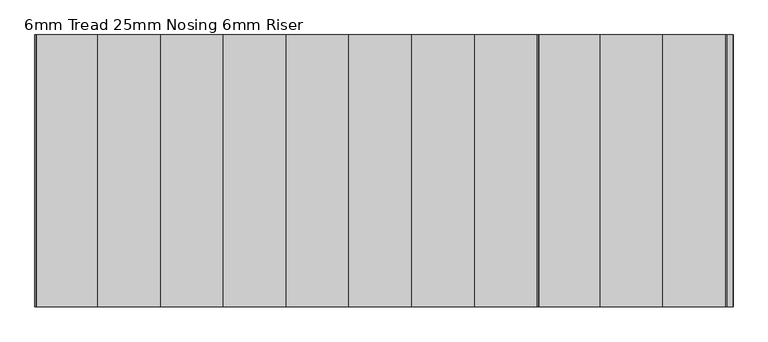
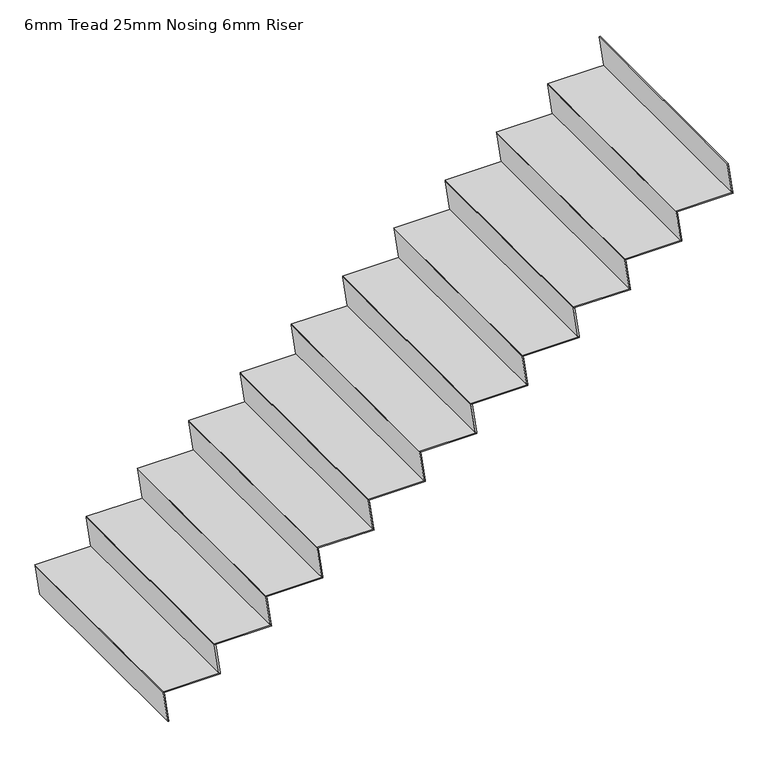
"""IFC4 building model written with IfcOpenShell, lengths in millimetres: stair flight geometry, 6mm Tread 25mm Nosing 6mm Riser."""

from ifc_helpers import new_model, si_unit, origin, place, context, project, spatial, faceted_brep, source, transform, mapped, element, save


def stair_flight_6mm_tread_25mm_nosing_6mm_riser_076b4cba(model_context):
    return source(origin(), model_context, "Body", "Brep", [
        faceted_brep([(-16043.9400908, 12030.4345331, 26529.4117647), (-16043.0900908, 12030.4345331, 26523.4117647), (-16043.0900908, 13220.4345331, 26523.4117647), (-16043.9400908, 13220.4345331, 26529.4117647), (-16350.0, 13220.4345331, 26529.4117647), (-16350.0, 12030.4345331, 26529.4117647), (-16349.15, 12030.4345331, 26523.4117647), (-16349.15, 13220.4345331, 26523.4117647)], [[[0, 1, 2, 3]], [[3, 4, 5, 0]], [[2, 1, 6, 7]], [[4, 3, 2, 7]], [[0, 5, 6, 1]], [[5, 4, 7, 6]]]),
        faceted_brep([(-16349.15, 12030.4345331, 26523.4117647), (-16325.0, 12030.4345331, 26352.9411765), (-16318.9400908, 12030.4345331, 26352.9411765), (-16343.0900908, 12030.4345331, 26523.4117647), (-16349.15, 13220.4345331, 26523.4117647), (-16343.0900908, 13220.4345331, 26523.4117647), (-16318.9400908, 13220.4345331, 26352.9411765), (-16325.0, 13220.4345331, 26352.9411765)], [[[0, 1, 2, 3]], [[4, 5, 6, 7]], [[1, 0, 4, 7]], [[2, 1, 7, 6]], [[3, 2, 6, 5]], [[0, 3, 5, 4]]]),
        faceted_brep([(-16074.15, 12030.4345331, 26699.8823529), (-16050.0, 12030.4345331, 26529.4117647), (-16043.9400908, 12030.4345331, 26529.4117647), (-16068.0900908, 12030.4345331, 26699.8823529), (-16074.15, 13220.4345331, 26699.8823529), (-16068.0900908, 13220.4345331, 26699.8823529), (-16043.9400908, 13220.4345331, 26529.4117647), (-16050.0, 13220.4345331, 26529.4117647)], [[[0, 1, 2, 3]], [[4, 5, 6, 7]], [[1, 0, 4, 7]], [[2, 1, 7, 6]], [[3, 2, 6, 5]], [[0, 3, 5, 4]]]),
        faceted_brep([(-15768.9400908, 13220.4345331, 26705.8823529), (-16075.0, 13220.4345331, 26705.8823529), (-16075.0, 12030.4345331, 26705.8823529), (-15768.9400908, 12030.4345331, 26705.8823529), (-15768.0900908, 13220.4345331, 26699.8823529), (-15768.0900908, 12030.4345331, 26699.8823529), (-16074.15, 12030.4345331, 26699.8823529), (-16074.15, 13220.4345331, 26699.8823529)], [[[0, 1, 2, 3]], [[4, 5, 6, 7]], [[1, 0, 4, 7]], [[3, 2, 6, 5]], [[3, 5, 4, 0]], [[2, 1, 7, 6]]]),
        faceted_brep([(-15799.15, 12030.4345331, 26876.3529412), (-15775.0, 12030.4345331, 26705.8823529), (-15768.9400908, 12030.4345331, 26705.8823529), (-15793.0900908, 12030.4345331, 26876.3529412), (-15799.15, 13220.4345331, 26876.3529412), (-15793.0900908, 13220.4345331, 26876.3529412), (-15768.9400908, 13220.4345331, 26705.8823529), (-15775.0, 13220.4345331, 26705.8823529)], [[[0, 1, 2, 3]], [[4, 5, 6, 7]], [[1, 0, 4, 7]], [[2, 1, 7, 6]], [[3, 2, 6, 5]], [[0, 3, 5, 4]]]),
        faceted_brep([(-15493.9400908, 13220.4345331, 26882.3529412), (-15800.0, 13220.4345331, 26882.3529412), (-15800.0, 12030.4345331, 26882.3529412), (-15493.9400908, 12030.4345331, 26882.3529412), (-15493.0900908, 13220.4345331, 26876.3529412), (-15493.0900908, 12030.4345331, 26876.3529412), (-15799.15, 12030.4345331, 26876.3529412), (-15799.15, 13220.4345331, 26876.3529412)], [[[0, 1, 2, 3]], [[4, 5, 6, 7]], [[1, 0, 4, 7]], [[3, 2, 6, 5]], [[3, 5, 4, 0]], [[2, 1, 7, 6]]]),
        faceted_brep([(-15524.15, 12030.4345331, 27052.8235294), (-15500.0, 12030.4345331, 26882.3529412), (-15493.9400908, 12030.4345331, 26882.3529412), (-15518.0900908, 12030.4345331, 27052.8235294), (-15524.15, 13220.4345331, 27052.8235294), (-15518.0900908, 13220.4345331, 27052.8235294), (-15493.9400908, 13220.4345331, 26882.3529412), (-15500.0, 13220.4345331, 26882.3529412)], [[[0, 1, 2, 3]], [[4, 5, 6, 7]], [[1, 0, 4, 7]], [[2, 1, 7, 6]], [[3, 2, 6, 5]], [[0, 3, 5, 4]]]),
        faceted_brep([(-15218.9400908, 13220.4345331, 27058.8235294), (-15525.0, 13220.4345331, 27058.8235294), (-15525.0, 12030.4345331, 27058.8235294), (-15218.9400908, 12030.4345331, 27058.8235294), (-15218.0900908, 13220.4345331, 27052.8235294), (-15218.0900908, 12030.4345331, 27052.8235294), (-15524.15, 12030.4345331, 27052.8235294), (-15524.15, 13220.4345331, 27052.8235294)], [[[0, 1, 2, 3]], [[4, 5, 6, 7]], [[1, 0, 4, 7]], [[3, 2, 6, 5]], [[3, 5, 4, 0]], [[2, 1, 7, 6]]]),
        faceted_brep([(-15249.15, 12030.4345331, 27229.2941176), (-15225.0, 12030.4345331, 27058.8235294), (-15218.9400908, 12030.4345331, 27058.8235294), (-15243.0900908, 12030.4345331, 27229.2941176), (-15249.15, 13220.4345331, 27229.2941176), (-15243.0900908, 13220.4345331, 27229.2941176), (-15218.9400908, 13220.4345331, 27058.8235294), (-15225.0, 13220.4345331, 27058.8235294)], [[[0, 1, 2, 3]], [[4, 5, 6, 7]], [[1, 0, 4, 7]], [[2, 1, 7, 6]], [[3, 2, 6, 5]], [[0, 3, 5, 4]]]),
        faceted_brep([(-14943.9400908, 13220.4345331, 27235.2941176), (-15250.0, 13220.4345331, 27235.2941176), (-15250.0, 12030.4345331, 27235.2941176), (-14943.9400908, 12030.4345331, 27235.2941176), (-14943.0900908, 13220.4345331, 27229.2941176), (-14943.0900908, 12030.4345331, 27229.2941176), (-15249.15, 12030.4345331, 27229.2941176), (-15249.15, 13220.4345331, 27229.2941176)], [[[0, 1, 2, 3]], [[4, 5, 6, 7]], [[1, 0, 4, 7]], [[3, 2, 6, 5]], [[3, 5, 4, 0]], [[2, 1, 7, 6]]]),
        faceted_brep([(-14974.15, 12030.4345331, 27405.7647059), (-14950.0, 12030.4345331, 27235.2941176), (-14943.9400908, 12030.4345331, 27235.2941176), (-14968.0900908, 12030.4345331, 27405.7647059), (-14974.15, 13220.4345331, 27405.7647059), (-14968.0900908, 13220.4345331, 27405.7647059), (-14943.9400908, 13220.4345331, 27235.2941176), (-14950.0, 13220.4345331, 27235.2941176)], [[[0, 1, 2, 3]], [[4, 5, 6, 7]], [[1, 0, 4, 7]], [[2, 1, 7, 6]], [[3, 2, 6, 5]], [[0, 3, 5, 4]]]),
        faceted_brep([(-14668.9400908, 13220.4345331, 27411.7647059), (-14975.0, 13220.4345331, 27411.7647059), (-14975.0, 12030.4345331, 27411.7647059), (-14668.9400908, 12030.4345331, 27411.7647059), (-14668.0900908, 13220.4345331, 27405.7647059), (-14668.0900908, 12030.4345331, 27405.7647059), (-14974.15, 12030.4345331, 27405.7647059), (-14974.15, 13220.4345331, 27405.7647059)], [[[0, 1, 2, 3]], [[4, 5, 6, 7]], [[1, 0, 4, 7]], [[3, 2, 6, 5]], [[3, 5, 4, 0]], [[2, 1, 7, 6]]]),
        faceted_brep([(-14699.15, 12030.4345331, 27582.2352941), (-14675.0, 12030.4345331, 27411.7647059), (-14668.9400908, 12030.4345331, 27411.7647059), (-14693.0900908, 12030.4345331, 27582.2352941), (-14699.15, 13220.4345331, 27582.2352941), (-14693.0900908, 13220.4345331, 27582.2352941), (-14668.9400908, 13220.4345331, 27411.7647059), (-14675.0, 13220.4345331, 27411.7647059)], [[[0, 1, 2, 3]], [[4, 5, 6, 7]], [[1, 0, 4, 7]], [[2, 1, 7, 6]], [[3, 2, 6, 5]], [[0, 3, 5, 4]]]),
        faceted_brep([(-14393.9400908, 13220.4345331, 27588.2352941), (-14700.0, 13220.4345331, 27588.2352941), (-14700.0, 12030.4345331, 27588.2352941), (-14393.9400908, 12030.4345331, 27588.2352941), (-14393.0900908, 13220.4345331, 27582.2352941), (-14393.0900908, 12030.4345331, 27582.2352941), (-14699.15, 12030.4345331, 27582.2352941), (-14699.15, 13220.4345331, 27582.2352941)], [[[0, 1, 2, 3]], [[4, 5, 6, 7]], [[1, 0, 4, 7]], [[3, 2, 6, 5]], [[3, 5, 4, 0]], [[2, 1, 7, 6]]]),
        faceted_brep([(-14424.15, 12030.4345331, 27758.7058824), (-14400.0, 12030.4345331, 27588.2352941), (-14393.9400908, 12030.4345331, 27588.2352941), (-14418.0900908, 12030.4345331, 27758.7058824), (-14424.15, 13220.4345331, 27758.7058824), (-14418.0900908, 13220.4345331, 27758.7058824), (-14393.9400908, 13220.4345331, 27588.2352941), (-14400.0, 13220.4345331, 27588.2352941)], [[[0, 1, 2, 3]], [[4, 5, 6, 7]], [[1, 0, 4, 7]], [[2, 1, 7, 6]], [[3, 2, 6, 5]], [[0, 3, 5, 4]]]),
        faceted_brep([(-14118.9400908, 13220.4345331, 27764.7058824), (-14425.0, 13220.4345331, 27764.7058824), (-14425.0, 12030.4345331, 27764.7058824), (-14118.9400908, 12030.4345331, 27764.7058824), (-14118.0900908, 13220.4345331, 27758.7058824), (-14118.0900908, 12030.4345331, 27758.7058824), (-14424.15, 12030.4345331, 27758.7058824), (-14424.15, 13220.4345331, 27758.7058824)], [[[0, 1, 2, 3]], [[4, 5, 6, 7]], [[1, 0, 4, 7]], [[3, 2, 6, 5]], [[3, 5, 4, 0]], [[2, 1, 7, 6]]]),
        faceted_brep([(-14149.15, 12030.4345331, 27935.1764706), (-14125.0, 12030.4345331, 27764.7058824), (-14118.9400908, 12030.4345331, 27764.7058824), (-14143.0900908, 12030.4345331, 27935.1764706), (-14149.15, 13220.4345331, 27935.1764706), (-14143.0900908, 13220.4345331, 27935.1764706), (-14118.9400908, 13220.4345331, 27764.7058824), (-14125.0, 13220.4345331, 27764.7058824)], [[[0, 1, 2, 3]], [[4, 5, 6, 7]], [[1, 0, 4, 7]], [[2, 1, 7, 6]], [[3, 2, 6, 5]], [[0, 3, 5, 4]]]),
        faceted_brep([(-13843.9400908, 13220.4345331, 27941.1764706), (-14150.0, 13220.4345331, 27941.1764706), (-14150.0, 12030.4345331, 27941.1764706), (-13843.9400908, 12030.4345331, 27941.1764706), (-13843.0900908, 13220.4345331, 27935.1764706), (-13843.0900908, 12030.4345331, 27935.1764706), (-14149.15, 12030.4345331, 27935.1764706), (-14149.15, 13220.4345331, 27935.1764706)], [[[0, 1, 2, 3]], [[4, 5, 6, 7]], [[1, 0, 4, 7]], [[3, 2, 6, 5]], [[3, 5, 4, 0]], [[2, 1, 7, 6]]]),
        faceted_brep([(-13874.15, 12030.4345331, 28111.6470588), (-13850.0, 12030.4345331, 27941.1764706), (-13843.9400908, 12030.4345331, 27941.1764706), (-13868.0900908, 12030.4345331, 28111.6470588), (-13874.15, 13220.4345331, 28111.6470588), (-13868.0900908, 13220.4345331, 28111.6470588), (-13843.9400908, 13220.4345331, 27941.1764706), (-13850.0, 13220.4345331, 27941.1764706)], [[[0, 1, 2, 3]], [[4, 5, 6, 7]], [[1, 0, 4, 7]], [[2, 1, 7, 6]], [[3, 2, 6, 5]], [[0, 3, 5, 4]]]),
        faceted_brep([(-13568.9400908, 13220.4345331, 28117.6470588), (-13875.0, 13220.4345331, 28117.6470588), (-13875.0, 12030.4345331, 28117.6470588), (-13568.9400908, 12030.4345331, 28117.6470588), (-13568.0900908, 13220.4345331, 28111.6470588), (-13568.0900908, 12030.4345331, 28111.6470588), (-13874.15, 12030.4345331, 28111.6470588), (-13874.15, 13220.4345331, 28111.6470588)], [[[0, 1, 2, 3]], [[4, 5, 6, 7]], [[1, 0, 4, 7]], [[3, 2, 6, 5]], [[3, 5, 4, 0]], [[2, 1, 7, 6]]]),
        faceted_brep([(-13324.15, 12030.4345331, 28464.5882353), (-13300.0, 12030.4345331, 28294.1176471), (-13293.9400908, 12030.4345331, 28294.1176471), (-13318.0900908, 12030.4345331, 28464.5882353), (-13324.15, 13220.4345331, 28464.5882353), (-13318.0900908, 13220.4345331, 28464.5882353), (-13293.9400908, 13220.4345331, 28294.1176471), (-13300.0, 13220.4345331, 28294.1176471)], [[[0, 1, 2, 3]], [[4, 5, 6, 7]], [[1, 0, 4, 7]], [[2, 1, 7, 6]], [[3, 2, 6, 5]], [[0, 3, 5, 4]]]),
        faceted_brep([(-13599.15, 12030.4345331, 28288.1176471), (-13575.0, 12030.4345331, 28117.6470588), (-13568.9400908, 12030.4345331, 28117.6470588), (-13593.0900908, 12030.4345331, 28288.1176471), (-13599.15, 13220.4345331, 28288.1176471), (-13593.0900908, 13220.4345331, 28288.1176471), (-13568.9400908, 13220.4345331, 28117.6470588), (-13575.0, 13220.4345331, 28117.6470588)], [[[0, 1, 2, 3]], [[4, 5, 6, 7]], [[1, 0, 4, 7]], [[2, 1, 7, 6]], [[3, 2, 6, 5]], [[0, 3, 5, 4]]]),
        faceted_brep([(-13293.9400908, 13220.4345331, 28294.1176471), (-13325.0, 13220.4345331, 28294.1176471), (-13600.0, 13220.4345331, 28294.1176471), (-13600.0, 12030.4345331, 28294.1176471), (-13293.9400908, 12030.4345331, 28294.1176471), (-13293.0900908, 13220.4345331, 28288.1176471), (-13293.0900908, 12030.4345331, 28288.1176471), (-13599.15, 12030.4345331, 28288.1176471), (-13599.15, 13220.4345331, 28288.1176471), (-13325.0, 13220.4345331, 28288.1176471)], [[[0, 1, 2, 3, 4]], [[5, 6, 7, 8, 9]], [[1, 0, 5, 9]], [[2, 1, 9, 8]], [[4, 3, 7, 6]], [[4, 6, 5, 0]], [[3, 2, 8, 7]]]),
    ])


if __name__ == "__main__":
    model = new_model("IFC4")
    model_context = context("Model", 3, world=origin())
    ifc_project = project(units=[si_unit("LENGTHUNIT", "METRE", prefix="MILLI")], contexts=[model_context])
    site = spatial("IfcSite", under=ifc_project)
    building = spatial("IfcBuilding", under=site)
    placement = place(None, origin())
    stair_flight_6mm_tread_25mm_nosing_6mm_riser_shape = stair_flight_6mm_tread_25mm_nosing_6mm_riser_076b4cba(model_context)
    element("IfcStairFlight", 1, ObjectType="6mm Tread 25mm Nosing 6mm Riser", at=placement, inside=building, context=model_context, shape_type="MappedRepresentation", body=[
        mapped(stair_flight_6mm_tread_25mm_nosing_6mm_riser_shape, transform((0.0, 0.0, 0.0), x_axis=(1.0, 0.0, 0.0), y_axis=(0.0, 1.0, 0.0), z_axis=(0.0, 0.0, 1.0))),
    ])
    save(model, "model.ifc")

# Revit data of these elements
# Element 1 (IfcStairFlight, "6mm Tread 25mm Nosing 6mm Riser")
#   Materials on its faces: "Steel, Paint Finish, Dark Gray"
# Materials
#   "Steel, Paint Finish, Dark Gray": class "Metal", colour RGB 89 89 89, transparency 0, Description = "Steel, paint finish, dark gray, glossy", Cost = 0
